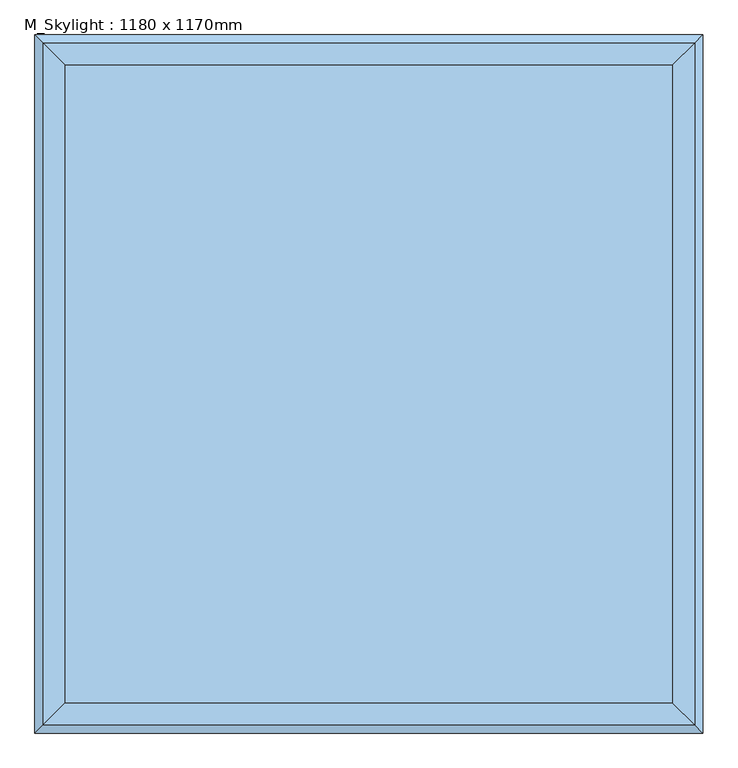
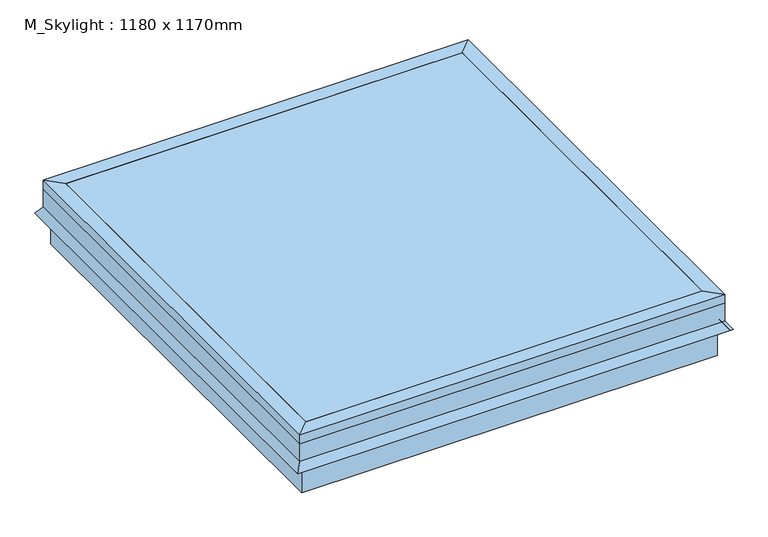
"""IFC4 building model written with IfcOpenShell, lengths in millimetres: window geometry, M_Skylight : 1180 x 1170mm."""

from ifc_helpers import new_model, si_unit, frame, origin, place, context, project, spatial, polyline, outline, extrude, faceted_brep, source, transform, mapped, element, save


def m_skylight_1180_x_1170mm_371bb450(model_context):
    return source(origin(), model_context, "Body", "SolidModel", [
        faceted_brep([(254.440073, 370.1040988, 4267.0), (279.840073, 395.5040988, 4267.0), (279.840073, -774.4959012, 4267.0), (254.440073, -749.0959012, 4267.0), (254.440073, 370.1040988, 4292.4), (254.440073, -749.0959012, 4292.4), (292.540073, 408.2040988, 4292.4), (292.540073, -787.1959012, 4292.4), (292.540073, 408.2040988, 4267.0), (292.540073, -787.1959012, 4267.0), (292.540073, 408.2040988, 4216.2), (292.540073, -787.1959012, 4216.2), (307.1089145, 422.7729403, 4195.3935381), (307.1089145, -801.7647427, 4195.3935381), (301.907299, 417.5713248, 4191.7513277), (301.907299, -796.5631272, 4191.7513277), (286.190073, 401.8540988, 4214.1978527), (286.190073, -780.8459012, 4214.1978527), (286.190073, 401.8540988, 4267.0), (286.190073, -780.8459012, 4267.0), (-838.159927, -774.4959012, 4267.0), (-812.759927, -749.0959012, 4267.0), (-812.759927, -749.0959012, 4292.4), (-850.859927, -787.1959012, 4292.4), (-850.859927, -787.1959012, 4267.0), (-850.859927, -787.1959012, 4216.2), (-865.4287685, -801.7647427, 4195.3935381), (-860.227153, -796.5631272, 4191.7513277), (-844.509927, -780.8459012, 4214.1978527), (-844.509927, -780.8459012, 4267.0), (-838.159927, 395.5040988, 4267.0), (-812.759927, 370.1040988, 4267.0), (-812.759927, 370.1040988, 4292.4), (-850.859927, 408.2040988, 4292.4), (-850.859927, 408.2040988, 4267.0), (-850.859927, 408.2040988, 4216.2), (-865.4287685, 422.7729403, 4195.3935381), (-860.227153, 417.5713248, 4191.7513277), (-844.509927, 401.8540988, 4214.1978527), (-844.509927, 401.8540988, 4267.0)], [[[0, 1, 2, 3]], [[4, 0, 3, 5]], [[6, 4, 5, 7]], [[8, 6, 7, 9]], [[10, 8, 9, 11]], [[12, 10, 11, 13]], [[14, 12, 13, 15]], [[16, 14, 15, 17]], [[18, 16, 17, 19]], [[1, 18, 19, 2]], [[3, 2, 20, 21]], [[5, 3, 21, 22]], [[7, 5, 22, 23]], [[9, 7, 23, 24]], [[11, 9, 24, 25]], [[13, 11, 25, 26]], [[15, 13, 26, 27]], [[17, 15, 27, 28]], [[19, 17, 28, 29]], [[2, 19, 29, 20]], [[21, 20, 30, 31]], [[22, 21, 31, 32]], [[23, 22, 32, 33]], [[24, 23, 33, 34]], [[25, 24, 34, 35]], [[26, 25, 35, 36]], [[27, 26, 36, 37]], [[28, 27, 37, 38]], [[29, 28, 38, 39]], [[20, 29, 39, 30]], [[31, 30, 1, 0]], [[32, 31, 0, 4]], [[33, 32, 4, 6]], [[34, 33, 6, 8]], [[35, 34, 8, 10]], [[36, 35, 10, 12]], [[37, 36, 12, 14]], [[38, 37, 14, 16]], [[39, 38, 16, 18]], [[30, 39, 18, 1]]]),
        faceted_brep([(279.840073, -774.4959012, 4267.0), (279.840073, -774.4959012, 4114.6), (279.840073, 395.5040988, 4114.6), (279.840073, 395.5040988, 4267.0), (254.440073, -749.0959012, 4267.0), (254.440073, 370.1040988, 4267.0), (254.440073, -749.0959012, 4241.6), (254.440073, 370.1040988, 4241.6), (235.390073, -730.0459012, 4241.6), (235.390073, 351.0540988, 4241.6), (235.390073, -730.0459012, 4114.6), (235.390073, 351.0540988, 4114.6), (-838.159927, 395.5040988, 4114.6), (-838.159927, 395.5040988, 4267.0), (-812.759927, 370.1040988, 4267.0), (-812.759927, 370.1040988, 4241.6), (-793.709927, 351.0540988, 4241.6), (-793.709927, 351.0540988, 4114.6), (-838.159927, -774.4959012, 4114.6), (-838.159927, -774.4959012, 4267.0), (-812.759927, -749.0959012, 4267.0), (-812.759927, -749.0959012, 4241.6), (-793.709927, -730.0459012, 4241.6), (-793.709927, -730.0459012, 4114.6)], [[[0, 1, 2, 3]], [[4, 0, 3, 5]], [[6, 4, 5, 7]], [[8, 6, 7, 9]], [[10, 8, 9, 11]], [[1, 10, 11, 2]], [[3, 2, 12, 13]], [[5, 3, 13, 14]], [[7, 5, 14, 15]], [[9, 7, 15, 16]], [[11, 9, 16, 17]], [[2, 11, 17, 12]], [[13, 12, 18, 19]], [[14, 13, 19, 20]], [[15, 14, 20, 21]], [[16, 15, 21, 22]], [[17, 16, 22, 23]], [[12, 17, 23, 18]], [[19, 18, 1, 0]], [[20, 19, 0, 4]], [[21, 20, 4, 6]], [[22, 21, 6, 8]], [[23, 22, 8, 10]], [[18, 23, 10, 1]]]),
        extrude(outline(polyline([(254.440073, -749.0959012), (-812.759927, -749.0959012), (-812.759927, 370.1040988), (254.440073, 370.1040988), (254.440073, -749.0959012)])), frame((0.0, 0.0, 4286.05), z_axis=(0.0, 0.0, 1.0), x_axis=(1.0, 0.0, 0.0)), (0.0, 0.0, 1.0), 6.35),
    ])


if __name__ == "__main__":
    model = new_model("IFC4")
    model_context = context("Model", 3, world=origin())
    ifc_project = project(units=[si_unit("LENGTHUNIT", "METRE", prefix="MILLI")], contexts=[model_context])
    site = spatial("IfcSite", under=ifc_project)
    building = spatial("IfcBuilding", under=site)
    placement = place(None, origin())
    m_skylight_1180_x_1170mm_shape = m_skylight_1180_x_1170mm_371bb450(model_context)
    element("IfcWindow", 1, ObjectType="M_Skylight : 1180 x 1170mm", at=placement, inside=building, context=model_context, shape_type="MappedRepresentation", body=[
        mapped(m_skylight_1180_x_1170mm_shape, transform((0.0, 0.0, 0.0), x_axis=(1.0, 0.0, 0.0), y_axis=(0.0, 1.0, 0.0), z_axis=(0.0, 0.0, 1.0))),
    ])
    save(model, "model.ifc")

# Revit data of these elements
# Type "M_Skylight : 1180 x 1170mm"
#   Manufacturer = "Manufacturer"
#   Type Mark = "36"
#   Construction Type = "Construction Type"
#   AccessibilityPerformance = "AccessibilityPerformance"
#   CodePerformance = "CodePerformance"
#   ConfigurationType = "ConfigurationType"
#   ConstructionType = "ConstructionType"
#   FireRating = "FireRating"
#   GlazingAreaFraction = "GlazingAreaFraction"
#   OperationType = "OperationType"
#   Area = "Area"
#   Color = "Color"
#   Constituents = "Constituents"
#   Features = "Features"
#   Finish = "Finish"
#   Grade = "Grade"
#   Material = "Material"
#   ModelReference = "ModelReference"
#   NominalHeight = "NominalHeight"
#   NominalLength = "NominalLength"
#   NominalWidth = "NominalWidth"
#   ProductionYear = "ProductionYear"
#   Reference = "Reference"
#   Shape = "Shape"
#   Size = "Size"
#   SustainabilityPerformance = "SustainabilityPerformance"
#   WarrantyDescription = "WarrantyDescription"
#   WarrantyDurationLabor = "WarrantyDurationLabor"
#   WarrantyDurationParts = "WarrantyDurationParts"
#   WarrantyGuarantorLabor = "WarrantyGuarantorLabor"
#   WarrantyGuarantorParts = "WarrantyGuarantorParts"
#   ExpectedLife = "ExpectedLife"
#   ReplacementCost = "ReplacementCost"
#   AssetAccountingType = "FIXED"
#   ModelLabel = "ModelLabel"
#   Height = 1.170 m
#   Width = 1.118 m
#   Sash Material = Metal - Bronze, Light Brush
#   Glass Pane Material = Glass
#   Frame Material = Metal - Bronze, Light Brush
#   Type Comments = ""
# Element 1 (IfcWindow, "M_Skylight : 1180 x 1170mm")
#   Materials on its faces: "Metal - Bronze, Light Brush", "Glass"
# Materials
#   "Metal - Bronze, Light Brush": class "Metal", colour RGB 113 80 70, transparency 0
#   "Glass": class "Glass", colour RGB 0 128 192, transparency 0.9
